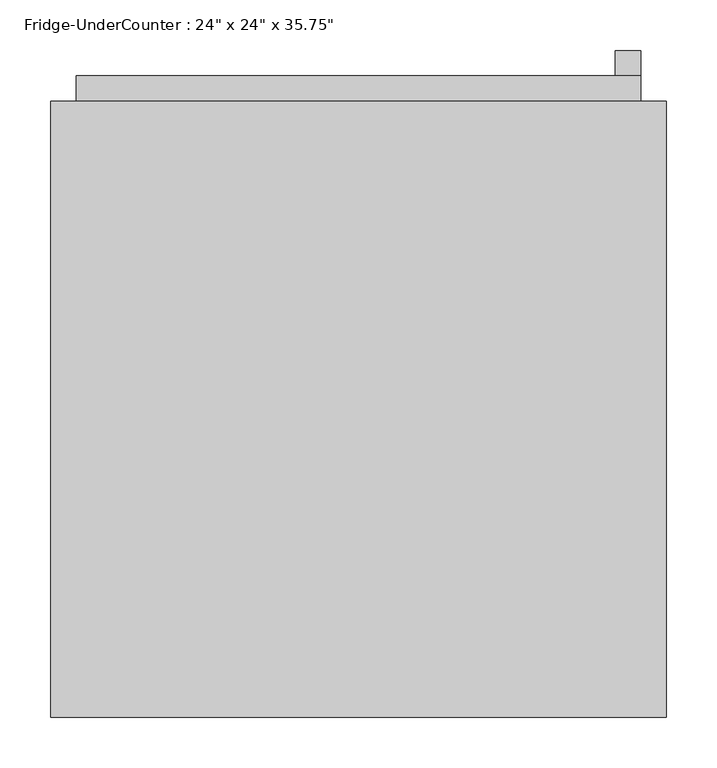
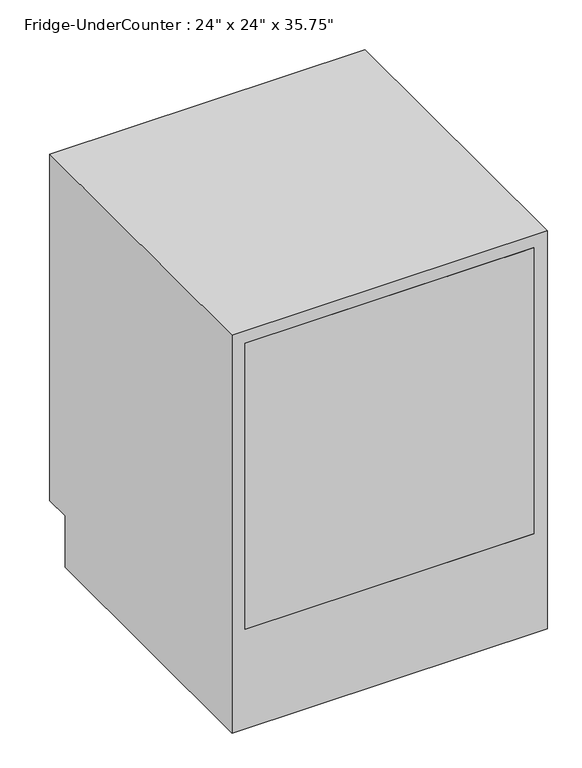
"""IFC4 building model written with IfcOpenShell, lengths in millimetres: proxy geometry."""

from ifc_helpers import new_model, si_unit, frame, origin, place, context, project, spatial, polyline, outline, extrude, faceted_brep, source, transform, mapped, element, save


def proxy_e0de9d9c(model_context):
    return source(origin(), model_context, "Body", "SolidModel", [
        extrude(outline(polyline([(388.969919, 596.9), (363.9849098, 596.9), (363.9849098, 749.3), (388.969919, 749.3), (388.969919, 596.9)]), holes=[polyline([(382.619919, 742.95), (369.1335899, 742.95), (369.1335899, 602.1696764), (382.619919, 602.1696764), (382.619919, 742.95)])]), frame((200.1988574, 0.0, 0.0), z_axis=(1.0, 0.0, 0.0), x_axis=(0.0, 1.0, 0.0)), (0.0, 0.0, 1.0), 25.4),
        extrude(outline(polyline([(193.8488574, 357.6349098), (193.8488574, 351.2849098), (-301.4511426, 351.2849098), (-301.4511426, 357.6349098), (193.8488574, 357.6349098)])), frame((0.0, 0.0, 234.95), z_axis=(0.0, 0.0, 1.0), x_axis=(1.0, 0.0, 0.0)), (0.0, 0.0, 1.0), 520.7),
        extrude(outline(polyline([(787.4, 225.5988574), (787.4, -333.2011426), (203.2, -333.2011426), (203.2, 225.5988574), (787.4, 225.5988574)]), holes=[polyline([(755.65, 193.8488574), (234.95, 193.8488574), (234.95, -301.4511426), (755.65, -301.4511426), (755.65, 193.8488574)])]), frame((0.0, 338.5849098, 0.0), z_axis=(0.0, 1.0, 0.0), x_axis=(0.0, 0.0, 1.0)), (0.0, 0.0, 1.0), 25.4),
        extrude(outline(polyline([(225.5988574, -245.6150902), (225.5988574, -271.0150902), (-333.2011426, -271.0150902), (-333.2011426, -245.6150902), (225.5988574, -245.6150902)])), frame((0.0, 0.0, 203.2), z_axis=(0.0, 0.0, 1.0), x_axis=(1.0, 0.0, 0.0)), (0.0, 0.0, 1.0), 584.2),
        faceted_brep([(250.9988574, 338.5849098, 812.8), (250.9988574, 338.5849098, 104.8297723), (-358.6011426, 338.5849098, 104.8297723), (-358.6011426, 338.5849098, 812.8), (225.5988574, 338.5849098, 787.4), (-333.2011426, 338.5849098, 787.4), (-333.2011426, 338.5849098, 203.2), (225.5988574, 338.5849098, 203.2), (250.9988574, -271.0150902, 812.8), (-358.6011426, -271.0150902, 812.8), (-358.6011426, -271.0150902, 0.0), (250.9988574, -271.0150902, 0.0), (225.5988574, -271.0150902, 787.4), (225.5988574, -271.0150902, 203.2), (-333.2011426, -271.0150902, 203.2), (-333.2011426, -271.0150902, 787.4), (-358.6011426, 287.7849098, 104.8297723), (-358.6011426, 287.7849098, 0.0), (250.9988574, 287.7849098, 0.0), (250.9988574, 287.7849098, 104.8297723)], [[[0, 1, 2, 3], [4, 5, 6, 7]], [[8, 9, 10, 11], [12, 13, 14, 15]], [[3, 9, 8, 0]], [[9, 3, 2, 16, 17, 10]], [[10, 17, 18, 11]], [[11, 18, 19, 1, 0, 8]], [[7, 13, 12, 4]], [[6, 14, 13, 7]], [[5, 15, 14, 6]], [[4, 12, 15, 5]], [[19, 18, 17, 16]], [[16, 2, 1, 19]]]),
    ])


if __name__ == "__main__":
    model = new_model("IFC4")
    model_context = context("Model", 3, world=origin())
    ifc_project = project(units=[si_unit("LENGTHUNIT", "METRE", prefix="MILLI")], contexts=[model_context])
    site = spatial("IfcSite", under=ifc_project)
    building = spatial("IfcBuilding", under=site)
    placement = place(None, origin())
    proxy_shape = proxy_e0de9d9c(model_context)
    element("IfcBuildingElementProxy", 1, Name="Fridge-UnderCounter : 24\" x 24\" x 35.75\"", ObjectType="Fridge-UnderCounter : 24\" x 24\" x 35.75\"", at=placement, inside=building, context=model_context, shape_type="MappedRepresentation", body=[
        mapped(proxy_shape, transform((0.0, 0.0, 0.0), x_axis=(1.0, 0.0, 0.0), y_axis=(0.0, 1.0, 0.0), z_axis=(0.0, 0.0, 1.0))),
    ])
    save(model, "model.ifc")

# Revit data of these elements
# Type "Fridge-UnderCounter : 24\" x 24\" x 35.75\""
#   Depth = 2' - 0"
#   Height = 2' - 8"
#   Width = 2' - 0"
#   Finish = Speciality Equipment
# Element 1 (IfcBuildingElementProxy, "Fridge-UnderCounter : 24\" x 24\" x 35.75\"")
#   Materials on its faces: "Speciality Equipment", "Steel"
# Materials
#   "Speciality Equipment": class "Generic", colour RGB 255 255 255, transparency 0, Cost = 0
#   "Steel": class "Metal", colour RGB 127 127 127, transparency 0
